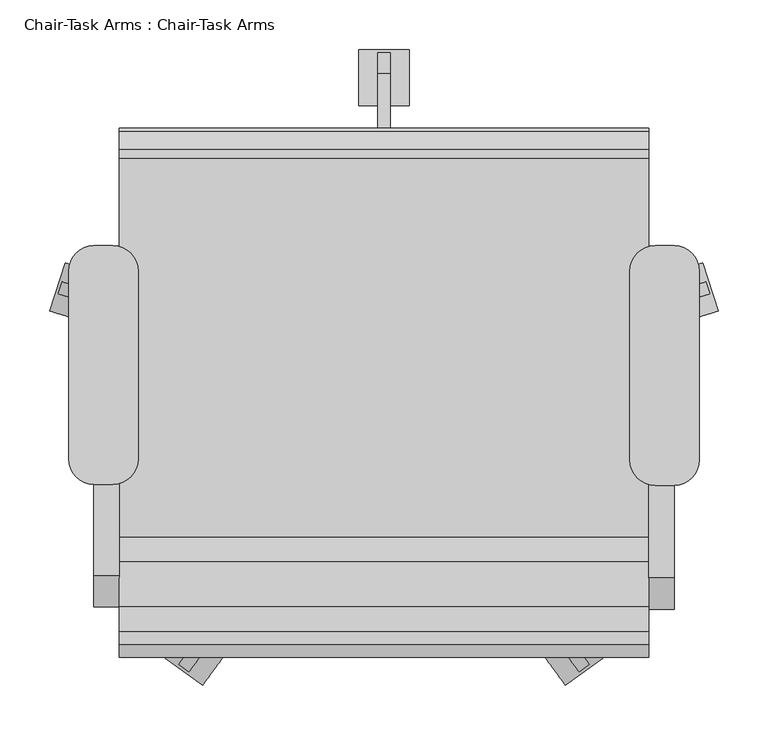
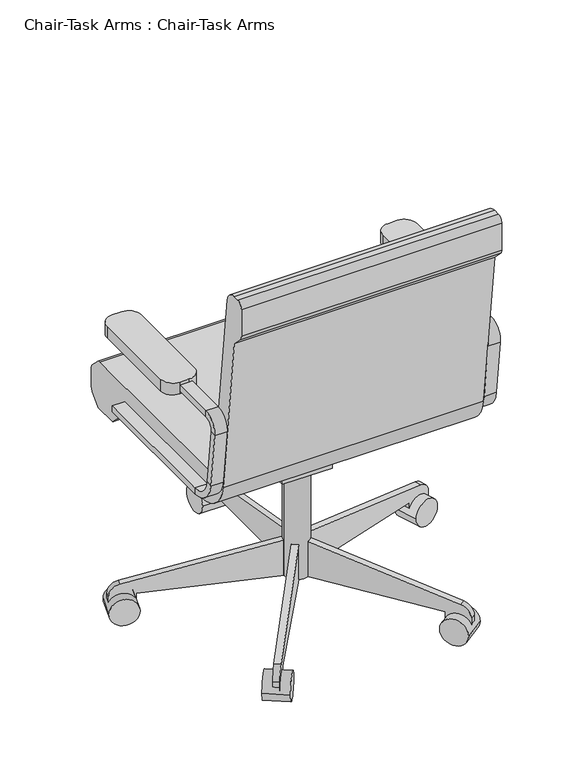
"""IFC4 building model written with IfcOpenShell, lengths in millimetres: furniture geometry, Chair-Task Arms : Chair-Task Arms."""

from ifc_helpers import new_model, si_unit, point, frame, frame_2d, origin, place, context, project, spatial, polyline, circle_curve, trimmed, segment, composite_curve, outline, extrude, source, transform, mapped, element, save
from ifc_brep_helpers import plane_surface, cylinder_surface, revolved_surface, advanced_brep


def chair_task_arms_chair_task_arms_8297d889(model_context):
    return source(origin(), model_context, "Body", "SolidModel", [
        extrude(outline(composite_curve([segment(polyline([(433.0908197, -74.2028048), (414.0408197, -74.2028048)]), True, "CONTINUOUS"), segment(trimmed(circle_curve(frame_2d((414.0408197, -48.8028048)), 25.4), [point((414.0408197, -74.2028048))], [point((388.6408197, -48.8028048))], False, "CARTESIAN"), True, "CONTINUOUS"), segment(polyline([(388.6408197, -48.8028048), (388.6408197, 141.6319091)]), True, "CONTINUOUS"), segment(trimmed(circle_curve(frame_2d((414.0408197, 141.6319091)), 25.4), [point((388.6408197, 141.6319091))], [point((414.0408197, 167.0319091))], False, "CARTESIAN"), True, "CONTINUOUS"), segment(polyline([(414.0408197, 167.0319091), (433.0908197, 167.0319091)]), True, "CONTINUOUS"), segment(trimmed(circle_curve(frame_2d((433.0908197, 141.6319091)), 25.4), [point((433.0908197, 167.0319091))], [point((458.4908197, 141.6319091))], False, "CARTESIAN"), True, "CONTINUOUS"), segment(polyline([(458.4908197, 141.6319091), (458.4908197, -48.8028048)]), True, "CONTINUOUS"), segment(trimmed(circle_curve(frame_2d((433.0908197, -48.8028048)), 25.4), [point((458.4908197, -48.8028048))], [point((433.0908197, -74.2028048))], False, "CARTESIAN"), True, "CONTINUOUS")], self_intersect=False)), frame((0.0, 0.0, 596.9), z_axis=(0.0, 0.0, 1.0), x_axis=(1.0, 0.0, 0.0)), (0.0, 0.0, 1.0), 25.4),
        extrude(outline(composite_curve([segment(polyline([(-132.0591803, -73.1575984), (-151.1091803, -73.1575984)]), True, "CONTINUOUS"), segment(trimmed(circle_curve(frame_2d((-151.1091803, -47.7575984)), 25.4), [point((-151.1091803, -73.1575984))], [point((-176.5091803, -47.7575984))], False, "CARTESIAN"), True, "CONTINUOUS"), segment(polyline([(-176.5091803, -47.7575984), (-176.5091803, 141.6319091)]), True, "CONTINUOUS"), segment(trimmed(circle_curve(frame_2d((-151.1091803, 141.6319091)), 25.4), [point((-176.5091803, 141.6319091))], [point((-151.1091803, 167.0319091))], False, "CARTESIAN"), True, "CONTINUOUS"), segment(polyline([(-151.1091803, 167.0319091), (-132.0591803, 167.0319091)]), True, "CONTINUOUS"), segment(trimmed(circle_curve(frame_2d((-132.0591803, 141.6319091)), 25.4), [point((-132.0591803, 167.0319091))], [point((-106.6591803, 141.6319091))], False, "CARTESIAN"), True, "CONTINUOUS"), segment(polyline([(-106.6591803, 141.6319091), (-106.6591803, -47.7575984)]), True, "CONTINUOUS"), segment(trimmed(circle_curve(frame_2d((-132.0591803, -47.7575984)), 25.4), [point((-106.6591803, -47.7575984))], [point((-132.0591803, -73.1575984))], False, "CARTESIAN"), True, "CONTINUOUS")], self_intersect=False)), frame((0.0, 0.0, 596.9), z_axis=(0.0, 0.0, 1.0), x_axis=(1.0, 0.0, 0.0)), (0.0, 0.0, 1.0), 25.4),
        advanced_brep(
        [(-151.1091803, 167.0319091, 412.75), (-151.1091803, 167.0319091, 425.45), (-125.7091803, 167.0319091, 425.45), (-125.7091803, 167.0319091, 412.75), (-151.1091803, -126.2388651, 412.75), (-151.1091803, -126.2388651, 425.45), (-125.7091803, -126.2388651, 425.45), (-125.7091803, -126.2388651, 412.75), (-151.1091803, -170.3844094, 464.7064065), (-151.1091803, -182.9974221, 463.2225227), (-125.7091803, -170.3844094, 464.7064065), (-125.7091803, -182.9974221, 463.2225227), (-151.1091803, -196.7936301, 580.4902904), (-151.1091803, -184.1806174, 581.9741742), (-125.7091803, -184.1806174, 581.9741742), (-125.7091803, -196.7936301, 580.4902904), (-151.1091803, -165.2610984, 603.25), (-151.1091803, -165.2610984, 615.95), (-125.7091803, -165.2610984, 603.25), (-125.7091803, -165.2610984, 615.95), (-151.1091803, 18.9459016, 615.95), (-125.7091803, 18.9459016, 615.95), (-125.7091803, 18.9459016, 603.25), (-151.1091803, 18.9459016, 603.25)],
        [
            (0, 1),
            (1, 2),
            (2, 3),
            (3, 0),
            (0, 4),
            (4, 5),
            (5, 1),
            (5, 6),
            (6, 2),
            (6, 7),
            (7, 3),
            (7, 4),
            (8, 5, circle_curve(frame((-151.1091803, -126.2388651, 469.9), z_axis=(1.0, 0.0, 0.0), x_axis=(0.0, 0.0, -1.0)), 44.45)),
            (4, 9, circle_curve(frame((-151.1091803, -126.2388651, 469.9), z_axis=(-1.0, 0.0, 0.0), x_axis=(0.0, 0.0, -1.0)), 57.15)),
            (9, 8),
            (10, 6, circle_curve(frame((-125.7091803, -126.2388651, 469.9), z_axis=(1.0, 0.0, 0.0), x_axis=(0.0, 0.0, -1.0)), 44.45)),
            (8, 10),
            (11, 7, circle_curve(frame((-125.7091803, -126.2388651, 469.9), z_axis=(1.0, 0.0, 0.0), x_axis=(0.0, 0.0, -1.0)), 57.15)),
            (10, 11),
            (11, 9),
            (9, 12),
            (12, 13),
            (13, 8),
            (13, 14),
            (14, 10),
            (14, 15),
            (15, 11),
            (15, 12),
            (16, 13, circle_curve(frame((-151.1091803, -165.2610984, 584.2), z_axis=(1.0, 0.0, 0.0), x_axis=(0.0, -0.993150604322877, -0.11684124756739026)), 19.05)),
            (12, 17, circle_curve(frame((-151.1091803, -165.2610984, 584.2), z_axis=(-1.0, 0.0, 0.0), x_axis=(0.0, -0.993150604322877, -0.11684124756739026)), 31.75)),
            (17, 16),
            (18, 14, circle_curve(frame((-125.7091803, -165.2610984, 584.2), z_axis=(1.0, 0.0, 0.0), x_axis=(0.0, -0.993150604322877, -0.11684124756739026)), 19.05)),
            (16, 18),
            (19, 15, circle_curve(frame((-125.7091803, -165.2610984, 584.2), z_axis=(1.0, 0.0, 0.0), x_axis=(0.0, -0.993150604322877, -0.11684124756739026)), 31.75)),
            (18, 19),
            (19, 17),
            (20, 21),
            (21, 22),
            (22, 23),
            (23, 20),
            (17, 20),
            (23, 16),
            (22, 18),
            (21, 19),
        ],
        [
            plane_surface(frame((-152.608212, 167.0319091, 419.1), z_axis=(0.0, 1.0, 0.0), x_axis=(0.0, 0.0, -1.0))),
            plane_surface(frame((-151.1091803, 167.0319091, 412.75), z_axis=(-1.0, 0.0, 0.0), x_axis=(0.0, -1.0, 0.0))),
            plane_surface(frame((-151.1091803, 167.0319091, 425.45), z_axis=(0.0, 0.0, 1.0), x_axis=(0.0, -1.0, 0.0))),
            plane_surface(frame((-125.7091803, 167.0319091, 425.45), z_axis=(1.0, 0.0, 0.0), x_axis=(0.0, -1.0, 0.0))),
            plane_surface(frame((-125.7091803, 167.0319091, 412.75), z_axis=(0.0, 0.0, -1.0), x_axis=(0.0, -1.0, 0.0))),
            plane_surface(frame((-151.1091803, -126.2388651, 469.9), z_axis=(-1.0, 0.0, 0.0), x_axis=(0.0, 0.0, -1.0))),
            revolved_surface(polyline([(-151.1091803, -126.2388651, 425.45), (-125.7091803, -126.2388651, 425.45)]), (-138.4091803, -126.2388651, 469.9), (-1.0, 0.0, 0.0)),
            plane_surface(frame((-125.7091803, -126.2388651, 469.9), z_axis=(1.0, 0.0, 0.0), x_axis=(0.0, 0.0, -1.0))),
            cylinder_surface(frame((-138.4091803, -126.2388651, 469.9), z_axis=(-1.0, 0.0, 0.0), x_axis=(0.0, 0.0, -1.0)), 57.15),
            plane_surface(frame((-151.1091803, -182.9974221, 463.2225227), z_axis=(-1.0, 0.0, 0.0), x_axis=(0.0, -0.11684124756738562, 0.9931506043228776))),
            plane_surface(frame((-151.1091803, -170.3844094, 464.7064065), z_axis=(0.0, 0.9931506043228776, 0.11684124756738562), x_axis=(0.0, -0.11684124756738562, 0.9931506043228776))),
            plane_surface(frame((-125.7091803, -170.3844094, 464.7064065), z_axis=(1.0, 0.0, 0.0), x_axis=(0.0, -0.11684124756738562, 0.9931506043228776))),
            plane_surface(frame((-125.7091803, -182.9974221, 463.2225227), z_axis=(0.0, -0.9931506043228776, -0.11684124756738562), x_axis=(0.0, -0.11684124756738562, 0.9931506043228776))),
            plane_surface(frame((-151.1091803, -165.2610984, 584.2), z_axis=(-1.0, 0.0, 0.0), x_axis=(0.0, -0.993150604322877, -0.11684124756739026))),
            revolved_surface(polyline([(-151.1091803, -184.1806174123508, 581.9741742338413), (-125.7091803, -184.1806174123508, 581.9741742338413)]), (-138.4091803, -165.2610984, 584.2), (-1.0, 0.0, 0.0)),
            plane_surface(frame((-125.7091803, -165.2610984, 584.2), z_axis=(1.0, 0.0, 0.0), x_axis=(0.0, -0.993150604322877, -0.11684124756739026))),
            cylinder_surface(frame((-138.4091803, -165.2610984, 584.2), z_axis=(-1.0, 0.0, 0.0), x_axis=(0.0, -0.993150604322877, -0.11684124756739026)), 31.75),
            plane_surface(frame((-152.608212, 18.9459016, 609.6), z_axis=(0.0, 1.0, 0.0), x_axis=(0.0, 0.0, 1.0))),
            plane_surface(frame((-151.1091803, -165.2610984, 615.95), z_axis=(-1.0, 0.0, 0.0), x_axis=(0.0, 1.0, 0.0))),
            plane_surface(frame((-151.1091803, -165.2610984, 603.25), z_axis=(0.0, 0.0, -1.0), x_axis=(0.0, 1.0, 0.0))),
            plane_surface(frame((-125.7091803, -165.2610984, 603.25), z_axis=(1.0, 0.0, 0.0), x_axis=(0.0, 1.0, 0.0))),
            plane_surface(frame((-125.7091803, -165.2610984, 615.95), z_axis=(0.0, 0.0, 1.0), x_axis=(0.0, 1.0, 0.0))),
        ],
        [
            (0, [[1, 2, 3, 4]]),
            (1, [[-1, 5, 6, 7]]),
            (2, [[-2, -7, 8, 9]]),
            (3, [[-3, -9, 10, 11]]),
            (4, [[-4, -11, 12, -5]]),
            (5, [[13, -6, 14, 15]]),
            (6, [[16, -8, -13, 17]]),
            (7, [[18, -10, -16, 19]]),
            (8, [[-14, -12, -18, 20]]),
            (9, [[-15, 21, 22, 23]]),
            (10, [[-17, -23, 24, 25]]),
            (11, [[-19, -25, 26, 27]]),
            (12, [[-20, -27, 28, -21]]),
            (13, [[29, -22, 30, 31]]),
            (14, [[32, -24, -29, 33]]),
            (15, [[34, -26, -32, 35]]),
            (16, [[-30, -28, -34, 36]]),
            (17, [[37, 38, 39, 40]]),
            (18, [[-31, 41, -40, 42]]),
            (19, [[-33, -42, -39, 43]]),
            (20, [[-35, -43, -38, 44]]),
            (21, [[-36, -44, -37, -41]]),
        ],
    ),
        advanced_brep(
        [(433.0908197, 167.0319091, 425.45), (433.0908197, 167.0319091, 412.75), (407.6908197, 167.0319091, 412.75), (407.6908197, 167.0319091, 425.45), (433.0908197, -128.329278, 425.45), (433.0908197, -128.329278, 412.75), (407.6908197, -128.329278, 412.75), (407.6908197, -128.329278, 425.45), (433.0908197, -185.0878351, 463.2225227), (433.0908197, -172.4748224, 464.7064065), (407.6908197, -185.0878351, 463.2225227), (407.6908197, -172.4748224, 464.7064065), (433.0908197, -186.2710303, 581.9741742), (433.0908197, -198.884043, 580.4902904), (407.6908197, -198.884043, 580.4902904), (407.6908197, -186.2710303, 581.9741742), (433.0908197, -167.3515113, 615.95), (433.0908197, -167.3515113, 603.25), (407.6908197, -167.3515113, 615.95), (407.6908197, -167.3515113, 603.25), (433.0908197, 18.9459016, 603.25), (407.6908197, 18.9459016, 603.25), (407.6908197, 18.9459016, 615.95), (433.0908197, 18.9459016, 615.95)],
        [
            (0, 1),
            (1, 2),
            (2, 3),
            (3, 0),
            (0, 4),
            (4, 5),
            (5, 1),
            (5, 6),
            (6, 2),
            (6, 7),
            (7, 3),
            (7, 4),
            (8, 5, circle_curve(frame((433.0908197, -128.329278, 469.9), z_axis=(1.0, 0.0, 0.0), x_axis=(0.0, 0.0, -1.0)), 57.15)),
            (4, 9, circle_curve(frame((433.0908197, -128.329278, 469.9), z_axis=(-1.0, 0.0, 0.0), x_axis=(0.0, 0.0, -1.0)), 44.45)),
            (9, 8),
            (10, 6, circle_curve(frame((407.6908197, -128.329278, 469.9), z_axis=(1.0, 0.0, 0.0), x_axis=(0.0, 0.0, -1.0)), 57.15)),
            (8, 10),
            (11, 7, circle_curve(frame((407.6908197, -128.329278, 469.9), z_axis=(1.0, 0.0, 0.0), x_axis=(0.0, 0.0, -1.0)), 44.45)),
            (10, 11),
            (11, 9),
            (9, 12),
            (12, 13),
            (13, 8),
            (13, 14),
            (14, 10),
            (14, 15),
            (15, 11),
            (15, 12),
            (16, 13, circle_curve(frame((433.0908197, -167.3515113, 584.2), z_axis=(1.0, 0.0, 0.0), x_axis=(0.0, -0.9931506043228767, -0.1168412475673929)), 31.75)),
            (12, 17, circle_curve(frame((433.0908197, -167.3515113, 584.2), z_axis=(-1.0, 0.0, 0.0), x_axis=(0.0, -0.9931506043228767, -0.1168412475673929)), 19.05)),
            (17, 16),
            (18, 14, circle_curve(frame((407.6908197, -167.3515113, 584.2), z_axis=(1.0, 0.0, 0.0), x_axis=(0.0, -0.9931506043228767, -0.1168412475673929)), 31.75)),
            (16, 18),
            (19, 15, circle_curve(frame((407.6908197, -167.3515113, 584.2), z_axis=(1.0, 0.0, 0.0), x_axis=(0.0, -0.9931506043228767, -0.1168412475673929)), 19.05)),
            (18, 19),
            (19, 17),
            (20, 21),
            (21, 22),
            (22, 23),
            (23, 20),
            (17, 20),
            (23, 16),
            (22, 18),
            (21, 19),
        ],
        [
            plane_surface(frame((406.191788, 167.0319091, 419.1), z_axis=(0.0, 1.0, 0.0), x_axis=(0.0, 0.0, -1.0))),
            plane_surface(frame((433.0908197, 167.0319091, 425.45), z_axis=(1.0, 0.0, 0.0), x_axis=(0.0, -1.0, 0.0))),
            plane_surface(frame((433.0908197, 167.0319091, 412.75), z_axis=(0.0, 0.0, -1.0), x_axis=(0.0, -1.0, 0.0))),
            plane_surface(frame((407.6908197, 167.0319091, 412.75), z_axis=(-1.0, 0.0, 0.0), x_axis=(0.0, -1.0, 0.0))),
            plane_surface(frame((407.6908197, 167.0319091, 425.45), z_axis=(0.0, 0.0, 1.0), x_axis=(0.0, -1.0, 0.0))),
            plane_surface(frame((433.0908197, -128.329278, 469.9), z_axis=(1.0, 0.0, 0.0), x_axis=(0.0, 0.0, -1.0))),
            cylinder_surface(frame((420.3908197, -128.329278, 469.9), z_axis=(-1.0, 0.0, 0.0), x_axis=(0.0, 0.0, -1.0)), 57.15),
            plane_surface(frame((407.6908197, -128.329278, 469.9), z_axis=(-1.0, 0.0, 0.0), x_axis=(0.0, 0.0, -1.0))),
            revolved_surface(polyline([(407.6908197, -128.329278, 425.45), (433.0908197, -128.329278, 425.45)]), (420.3908197, -128.329278, 469.9), (-1.0, 0.0, 0.0)),
            plane_surface(frame((433.0908197, -172.4748224, 464.7064065), z_axis=(1.0, 0.0, 0.0), x_axis=(0.0, -0.11684124756738622, 0.9931506043228775))),
            plane_surface(frame((433.0908197, -185.0878351, 463.2225227), z_axis=(0.0, -0.9931506043228775, -0.11684124756738622), x_axis=(0.0, -0.11684124756738622, 0.9931506043228775))),
            plane_surface(frame((407.6908197, -185.0878351, 463.2225227), z_axis=(-1.0, 0.0, 0.0), x_axis=(0.0, -0.11684124756738622, 0.9931506043228775))),
            plane_surface(frame((407.6908197, -172.4748224, 464.7064065), z_axis=(0.0, 0.9931506043228775, 0.11684124756738622), x_axis=(0.0, -0.11684124756738622, 0.9931506043228775))),
            plane_surface(frame((433.0908197, -167.3515113, 584.2), z_axis=(1.0, 0.0, 0.0), x_axis=(0.0, -0.9931506043228767, -0.1168412475673929))),
            cylinder_surface(frame((420.3908197, -167.3515113, 584.2), z_axis=(-1.0, 0.0, 0.0), x_axis=(0.0, -0.9931506043228767, -0.1168412475673929)), 31.75),
            plane_surface(frame((407.6908197, -167.3515113, 584.2), z_axis=(-1.0, 0.0, 0.0), x_axis=(0.0, -0.9931506043228767, -0.1168412475673929))),
            revolved_surface(polyline([(407.6908197, -186.2710303123508, 581.9741742338412), (433.0908197, -186.2710303123508, 581.9741742338412)]), (420.3908197, -167.3515113, 584.2), (-1.0, 0.0, 0.0)),
            plane_surface(frame((406.191788, 18.9459016, 609.6), z_axis=(0.0, 1.0, 0.0), x_axis=(0.0, 0.0, 1.0))),
            plane_surface(frame((433.0908197, -167.3515113, 603.25), z_axis=(1.0, 0.0, 0.0), x_axis=(0.0, 1.0, 0.0))),
            plane_surface(frame((433.0908197, -167.3515113, 615.95), z_axis=(0.0, 0.0, 1.0), x_axis=(0.0, 1.0, 0.0))),
            plane_surface(frame((407.6908197, -167.3515113, 615.95), z_axis=(-1.0, 0.0, 0.0), x_axis=(0.0, 1.0, 0.0))),
            plane_surface(frame((407.6908197, -167.3515113, 603.25), z_axis=(0.0, 0.0, -1.0), x_axis=(0.0, 1.0, 0.0))),
        ],
        [
            (0, [[1, 2, 3, 4]]),
            (1, [[-1, 5, 6, 7]]),
            (2, [[-2, -7, 8, 9]]),
            (3, [[-3, -9, 10, 11]]),
            (4, [[-4, -11, 12, -5]]),
            (5, [[13, -6, 14, 15]]),
            (6, [[16, -8, -13, 17]]),
            (7, [[18, -10, -16, 19]]),
            (8, [[-14, -12, -18, 20]]),
            (9, [[-15, 21, 22, 23]]),
            (10, [[-17, -23, 24, 25]]),
            (11, [[-19, -25, 26, 27]]),
            (12, [[-20, -27, 28, -21]]),
            (13, [[29, -22, 30, 31]]),
            (14, [[32, -24, -29, 33]]),
            (15, [[34, -26, -32, 35]]),
            (16, [[-30, -28, -34, 36]]),
            (17, [[37, 38, 39, 40]]),
            (18, [[-31, 41, -40, 42]]),
            (19, [[-33, -42, -39, 43]]),
            (20, [[-35, -43, -38, 44]]),
            (21, [[-36, -44, -37, -41]]),
        ],
    ),
        extrude(outline(composite_curve([segment(trimmed(circle_curve(frame_2d((140.9908197, 18.9459016)), 25.4), [point((115.5908197, 18.9459016))], [point((166.3908197, 18.9459016))], False, "CARTESIAN"), True, "CONTINUOUS"), segment(trimmed(circle_curve(frame_2d((140.9908197, 18.9459016)), 25.4), [point((166.3908197, 18.9459016))], [point((115.5908197, 18.9459016))], False, "CARTESIAN"), True, "CONTINUOUS")], self_intersect=False)), frame((0.0, 0.0, 53.5835944), z_axis=(0.0, 0.0, 1.0), x_axis=(1.0, 0.0, 0.0)), (0.0, 0.0, 1.0), 330.5914056),
        extrude(outline(composite_curve([segment(trimmed(circle_curve(frame_2d((0.0, -28.2002727)), 28.2002727), [point((0.0, -56.4005455))], [point((0.0, 0.0))], False, "CARTESIAN"), True, "CONTINUOUS"), segment(trimmed(circle_curve(frame_2d((0.0, -28.2002727)), 28.2002727), [point((0.0, 0.0))], [point((0.0, -56.4005455))], False, "CARTESIAN"), True, "CONTINUOUS")], self_intersect=False)), frame((477.6203484, 101.6163254, 28.1835944), z_axis=(-0.3090169943749423, 0.9510565162951553, 0.0), x_axis=(0.0, 0.0, 1.0)), (0.0, 0.0, 1.0), 50.8),
        extrude(outline(composite_curve([segment(polyline([(-25.4, 0.0), (0.0, 0.0), (0.0, -50.8), (-24.303053, -50.8)]), True, "CONTINUOUS"), segment(trimmed(circle_curve(frame_2d((-24.303053, -25.4)), 25.4), [point((-24.303053, -50.8))], [point((-49.3171699, -29.8106637))], False, "CARTESIAN"), True, "CONTINUOUS"), segment(polyline([(-49.3171699, -29.8106637), (-101.6, 266.7), (-101.6, 292.1), (-25.4, 292.1), (-25.4, 0.0)]), True, "CONTINUOUS")], self_intersect=False)), frame((420.756686, 103.1705568, 28.1835944), z_axis=(-0.3090169943749423, 0.9510565162951553, 0.0), x_axis=(0.0, 0.0, -1.0)), (0.0, 0.0, 1.0), 12.7),
        extrude(outline(composite_curve([segment(trimmed(circle_curve(frame_2d((0.0, -28.2002727)), 28.2002727), [point((0.0, -56.4005455))], [point((0.0, 0.0))], False, "CARTESIAN"), True, "CONTINUOUS"), segment(trimmed(circle_curve(frame_2d((0.0, -28.2002727)), 28.2002727), [point((0.0, 0.0))], [point((0.0, -56.4005455))], False, "CARTESIAN"), True, "CONTINUOUS")], self_intersect=False)), frame((323.63931, -275.6612394, 28.1835944), z_axis=(0.8090169943749499, 0.5877852522924699, 0.0), x_axis=(0.0, 0.0, 1.0)), (0.0, 0.0, 1.0), 50.8),
        extrude(outline(composite_curve([segment(polyline([(-25.4, 0.0), (0.0, 0.0), (0.0, -50.8), (-24.303053, -50.8)]), True, "CONTINUOUS"), segment(trimmed(circle_curve(frame_2d((-24.303053, -25.3999999)), 25.4), [point((-24.303053, -50.8))], [point((-49.3171699, -29.8106636))], False, "CARTESIAN"), True, "CONTINUOUS"), segment(polyline([(-49.3171699, -29.8106636), (-101.6, 266.7), (-101.6, 292.1), (-25.4, 292.1), (-25.4, 0.0)]), True, "CONTINUOUS")], self_intersect=False)), frame((307.545634, -221.1003988, 28.1835944), z_axis=(0.8090169943749499, 0.5877852522924699, 0.0), x_axis=(0.0, 0.0, -1.0)), (0.0, 0.0, 1.0), 12.7),
        extrude(outline(composite_curve([segment(trimmed(circle_curve(frame_2d((0.0, -28.2002727)), 28.2002727), [point((0.0, -56.4005455))], [point((0.0, 0.0))], False, "CARTESIAN"), True, "CONTINUOUS"), segment(trimmed(circle_curve(frame_2d((0.0, -28.2002727)), 28.2002727), [point((0.0, 0.0))], [point((0.0, -56.4005455))], False, "CARTESIAN"), True, "CONTINUOUS")], self_intersect=False)), frame((-41.6576707, -275.6612394, 28.1835944), z_axis=(-0.8090169943749458, 0.5877852522924754, 0.0), x_axis=(0.0, 0.0, -1.0)), (0.0, 0.0, 1.0), 50.8),
        extrude(outline(composite_curve([segment(polyline([(25.4, 0.0), (25.4, 292.1), (101.6, 292.1), (101.6, 266.7), (49.3171699, -29.8106637)]), True, "CONTINUOUS"), segment(trimmed(circle_curve(frame_2d((24.303053, -25.3999999)), 25.4), [point((49.3171699, -29.8106637))], [point((24.303053, -50.8))], False, "CARTESIAN"), True, "CONTINUOUS"), segment(polyline([(24.303053, -50.8), (0.0, -50.8), (0.0, 0.0), (25.4, 0.0)]), True, "CONTINUOUS")], self_intersect=False)), frame((-25.5639946, -221.1003988, 28.1835944), z_axis=(-0.8090169943749459, 0.5877852522924754, 0.0), x_axis=(0.0, 0.0, 1.0)), (0.0, 0.0, 1.0), 12.7),
        extrude(outline(composite_curve([segment(trimmed(circle_curve(frame_2d((0.0, -28.2002727)), 28.2002727), [point((0.0, -56.4005454))], [point((0.0, 0.0))], False, "CARTESIAN"), True, "CONTINUOUS"), segment(trimmed(circle_curve(frame_2d((0.0, -28.2002727)), 28.2002727), [point((0.0, 0.0))], [point((0.0, -56.4005454))], False, "CARTESIAN"), True, "CONTINUOUS")], self_intersect=False)), frame((-195.638709, 101.6163254, 28.1835944), z_axis=(0.3090169943749487, 0.9510565162951532, 0.0), x_axis=(0.0, 0.0, -1.0)), (0.0, 0.0, 1.0), 50.8),
        extrude(outline(composite_curve([segment(polyline([(25.4, 0.0), (25.4, 292.1000001), (101.6, 292.1000001), (101.6, 266.7), (49.3171699, -29.8106636)]), True, "CONTINUOUS"), segment(trimmed(circle_curve(frame_2d((24.303053, -25.4)), 25.4), [point((49.3171699, -29.8106636))], [point((24.303053, -50.8))], False, "CARTESIAN"), True, "CONTINUOUS"), segment(polyline([(24.303053, -50.8), (0.0, -50.8), (0.0, 0.0), (25.4, 0.0)]), True, "CONTINUOUS")], self_intersect=False)), frame((-138.7750467, 103.1705568, 28.1835944), z_axis=(0.3090169943749487, 0.9510565162951532, 0.0), x_axis=(0.0, 0.0, 1.0)), (0.0, 0.0, 1.0), 12.7),
        extrude(outline(composite_curve([segment(trimmed(circle_curve(frame_2d((336.4459016, 28.1835944)), 28.2002727), [point((308.2456289, 28.1835944))], [point((364.6461744, 28.1835944))], False, "CARTESIAN"), True, "CONTINUOUS"), segment(trimmed(circle_curve(frame_2d((336.4459016, 28.1835944)), 28.2002727), [point((364.6461744, 28.1835944))], [point((308.2456289, 28.1835944))], False, "CARTESIAN"), True, "CONTINUOUS")], self_intersect=False)), frame((115.5908197, 0.0, 0.0), z_axis=(1.0, 0.0, 0.0), x_axis=(0.0, 1.0, 0.0)), (0.0, 0.0, 1.0), 50.8),
        extrude(outline(composite_curve([segment(polyline([(311.0459016, 53.5835944), (18.9459016, 53.5835944), (18.9459016, 129.7835944), (44.3459016, 129.7835944), (340.8565654, 77.5007643)]), True, "CONTINUOUS"), segment(trimmed(circle_curve(frame_2d((336.4459016, 52.4866474)), 25.4), [point((340.8565654, 77.5007643))], [point((361.8459016, 52.4866474))], False, "CARTESIAN"), True, "CONTINUOUS"), segment(polyline([(361.8459016, 52.4866474), (361.8459016, 28.1835944), (311.0459016, 28.1835944), (311.0459016, 53.5835944)]), True, "CONTINUOUS")], self_intersect=False)), frame((134.6408197, 0.0, 0.0), z_axis=(1.0, 0.0, 0.0), x_axis=(0.0, 1.0, 0.0)), (0.0, 0.0, 1.0), 12.7),
        extrude(outline(polyline([(69.7459016, 383.7835944), (69.7459016, 371.0835944), (18.9459016, 283.0954134), (-19.1540984, 283.0954134), (-19.1540984, 383.7835944), (69.7459016, 383.7835944)])), frame((90.1908197, 0.0, 0.0), z_axis=(1.0, 0.0, 0.0), x_axis=(0.0, 1.0, 0.0)), (0.0, 0.0, 1.0), 101.6),
        extrude(outline(composite_curve([segment(polyline([(-126.2050455, 457.2), (255.0102301, 457.2)]), True, "CONTINUOUS"), segment(trimmed(circle_curve(frame_2d((255.0102301, 444.5)), 12.7), [point((255.0102301, 457.2))], [point((263.9604301, 453.510212))], False, "CARTESIAN"), True, "CONTINUOUS"), segment(polyline([(263.9604301, 453.510212), (281.8961016, 435.6939999)]), True, "CONTINUOUS"), segment(trimmed(circle_curve(frame_2d((272.9459016, 426.6837879)), 12.7), [point((281.8961016, 435.6939999))], [point((285.6459016, 426.6837879))], False, "CARTESIAN"), True, "CONTINUOUS"), segment(polyline([(285.6459016, 426.6837879), (285.6459016, 391.6405184)]), True, "CONTINUOUS"), segment(trimmed(circle_curve(frame_2d((260.2459016, 391.6405184)), 25.4), [point((285.6459016, 391.6405184))], [point((278.2663256, 373.7401184))], False, "CARTESIAN"), True, "CONTINUOUS"), segment(polyline([(278.2663256, 373.7401184), (260.2470284, 355.6), (209.4470284, 355.6), (181.0744602, 383.7835944), (-107.1089978, 383.7835944)]), True, "CONTINUOUS"), segment(trimmed(circle_curve(frame_2d((-107.1089978, 459.9835944)), 76.2), [point((-107.1089978, 383.7835944))], [point((-182.7870738, 451.0802913))], False, "CARTESIAN"), True, "CONTINUOUS"), segment(polyline([(-182.7870738, 451.0802913), (-222.3540984, 787.4), (-244.0343545, 809.0802561)]), True, "CONTINUOUS"), segment(trimmed(circle_curve(frame_2d((-235.0540984, 818.0605122)), 12.7), [point((-244.0343545, 809.0802561))], [point((-247.7540984, 818.0605122))], False, "CARTESIAN"), True, "CONTINUOUS"), segment(polyline([(-247.7540984, 818.0605122), (-247.7540984, 876.3)]), True, "CONTINUOUS"), segment(trimmed(circle_curve(frame_2d((-235.0540984, 876.3)), 12.7), [point((-247.7540984, 876.3))], [point((-235.0540984, 889.0))], False, "CARTESIAN"), True, "CONTINUOUS"), segment(polyline([(-235.0540984, 889.0), (-222.1789239, 889.0)]), True, "CONTINUOUS"), segment(trimmed(circle_curve(frame_2d((-222.1789239, 863.6)), 25.4), [point((-222.1789239, 889.0))], [point((-196.9528985, 866.5677677))], False, "CARTESIAN"), True, "CONTINUOUS"), segment(polyline([(-196.9528985, 866.5677677), (-151.4310708, 479.6322323)]), True, "CONTINUOUS"), segment(trimmed(circle_curve(frame_2d((-126.2050455, 482.6)), 25.4), [point((-151.4310708, 479.6322323))], [point((-126.2050455, 457.2))], True, "CARTESIAN"), True, "CONTINUOUS")], self_intersect=False)), frame((-125.7091803, 0.0, 0.0), z_axis=(1.0, 0.0, 0.0), x_axis=(0.0, 1.0, 0.0)), (0.0, 0.0, 1.0), 533.4),
    ])


if __name__ == "__main__":
    model = new_model("IFC4")
    model_context = context("Model", 3, world=origin())
    ifc_project = project(units=[si_unit("LENGTHUNIT", "METRE", prefix="MILLI")], contexts=[model_context])
    site = spatial("IfcSite", under=ifc_project)
    building = spatial("IfcBuilding", under=site)
    placement = place(None, origin())
    chair_task_arms_chair_task_arms_shape = chair_task_arms_chair_task_arms_8297d889(model_context)
    element("IfcFurniture", 1, ObjectType="Chair-Task Arms : Chair-Task Arms", at=placement, inside=building, context=model_context, shape_type="MappedRepresentation", body=[
        mapped(chair_task_arms_chair_task_arms_shape, transform((0.0, 0.0, 0.0), x_axis=(1.0, 0.0, 0.0), y_axis=(0.0, 1.0, 0.0), z_axis=(0.0, 0.0, 1.0))),
    ])
    save(model, "model.ifc")

# Revit data of these elements
# Type "Chair-Task Arms : Chair-Task Arms"
#   Model = "CHTSK-095"
#   Manufacturer = "Furniture Concepts"
#   Type Mark = "CH-3"
#   Assembly Code = "E2020200"
#   Cost = 1095
#   Base Material = Plastic, Opaque Black
#   Caster Material = Plastic, Opaque Black
#   Seat/Back Material = Leather - Matte (Tan)
#   Default Elevation = 0
# Element 1 (IfcFurniture, "Chair-Task Arms : Chair-Task Arms")
#   Materials on its faces: "Plastic, Opaque Black", "Leather - Matte (Tan)"
# Materials
#   "Plastic, Opaque Black": class "Plastic", colour RGB 0 0 0, transparency 0, Description = "Plastic, generic, opaque black", Cost = 0
#   "Leather - Matte (Tan)": class "Generic", colour RGB 162 130 69, transparency 0, Cost = 0
